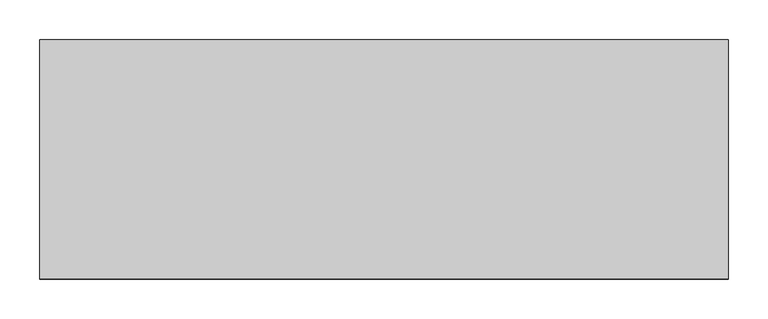
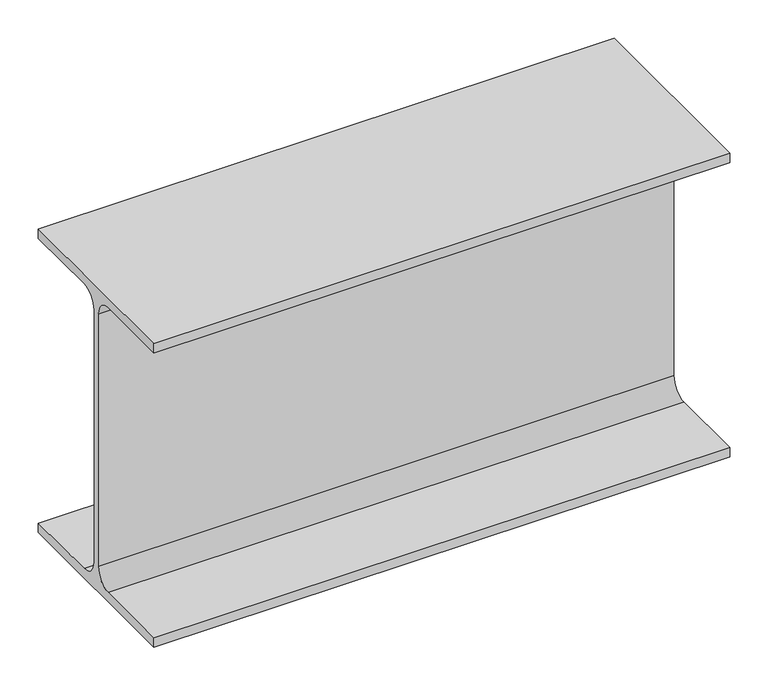
"""IFC4 building model written with IfcOpenShell, lengths in millimetres: beam geometry, 0912_Steel Framing_H-KSD3502 : H_SB_ASB_H-482x300x11x15."""

from ifc_helpers import new_model, si_unit, point, frame, frame_2d, origin, place, context, project, spatial, polyline, circle_curve, trimmed, segment, composite_curve, outline, extrude, source, transform, mapped, element, save


def beam_93cadcc3(model_context):
    return source(origin(), model_context, "Body", "SweptSolid", [
        extrude(outline(composite_curve([segment(polyline([(150.0, -226.0), (150.0, -241.0), (-150.0, -241.0), (-150.0, -226.0), (-31.5, -226.0)]), True, "CONTINUOUS"), segment(trimmed(circle_curve(frame_2d((-31.5, -200.0)), 26.0), [point((-31.5, -226.0))], [point((-5.5, -200.0))], True, "CARTESIAN"), True, "CONTINUOUS"), segment(polyline([(-5.5, -200.0), (-5.5, 200.0)]), True, "CONTINUOUS"), segment(trimmed(circle_curve(frame_2d((-31.5, 200.0)), 26.0), [point((-5.5, 200.0))], [point((-31.5, 226.0))], True, "CARTESIAN"), True, "CONTINUOUS"), segment(polyline([(-31.5, 226.0), (-150.0, 226.0), (-150.0, 241.0), (150.0, 241.0), (150.0, 226.0), (31.5, 226.0)]), True, "CONTINUOUS"), segment(trimmed(circle_curve(frame_2d((31.5, 200.0)), 26.0), [point((31.5, 226.0))], [point((5.5, 200.0))], True, "CARTESIAN"), True, "CONTINUOUS"), segment(polyline([(5.5, 200.0), (5.5, -200.0)]), True, "CONTINUOUS"), segment(trimmed(circle_curve(frame_2d((31.5, -200.0)), 26.0), [point((5.5, -200.0))], [point((31.5, -226.0))], True, "CARTESIAN"), True, "CONTINUOUS"), segment(polyline([(31.5, -226.0), (150.0, -226.0)]), True, "CONTINUOUS")], self_intersect=False)), frame((-431.8, 0.0, 0.0), z_axis=(1.0, 0.0, 0.0), x_axis=(0.0, 1.0, 0.0)), (0.0, 0.0, 1.0), 863.6),
    ])


if __name__ == "__main__":
    model = new_model("IFC4")
    model_context = context("Model", 3, world=origin())
    ifc_project = project(units=[si_unit("LENGTHUNIT", "METRE", prefix="MILLI")], contexts=[model_context])
    site = spatial("IfcSite", under=ifc_project)
    building = spatial("IfcBuilding", under=site)
    placement = place(None, origin())
    beam_shape = beam_93cadcc3(model_context)
    element("IfcBeam", 1, ObjectType="0912_Steel Framing_H-KSD3502 : H_SB_ASB_H-482x300x11x15", at=placement, inside=building, context=model_context, shape_type="MappedRepresentation", body=[
        mapped(beam_shape, transform((0.0, 0.0, 0.0), x_axis=(1.0, 0.0, 0.0), y_axis=(0.0, 1.0, 0.0), z_axis=(0.0, 0.0, 1.0))),
    ])
    save(model, "model.ifc")

# Revit data of these elements
# Type "0912_Steel Framing_H-KSD3502 : H_SB_ASB_H-482x300x11x15"
#   H_WM Code_1 = "S01AA001-00001 | Main Steel Structure Fabrication Work | Shelter/Building | Heavy Steel - Standard (Weight≥90KG/M) | Material: (   )"
#   H_WM Code_2 = "S03AA027-00001 | Main Steel Structure Erection Work | Shelter/Building | Heavy Steel (Weight≥90KG/M) | Material: (   )"
#   H_WM Code_3 = "S01AA010-00001 | Main Steel Structure Fabrication Work | Shelter/Building | Steel Painting/Coating | for Non-Fireproofed Steel Surface, Surface Preparation, Primer, Second & Final Coat | Material: (   )"
#   H_Q'ty Cal Type Tag = "SB-Q2"
#   Width = 30.0 cm
#   Web Thickness = 1.1 cm
#   Web Fillet = 2.6 cm
#   Warping Constant = 3680000.0 cm⁶
#   W = 0
#   Torsional Moment of Inertia = 88.2192 cm⁴
#   Section Area = 145.5 cm²
#   Plastic Modulus weak axis = 695.0 cm³
#   Plastic Modulus strong axis = 2790.0 cm³
#   Perimeter = 2.10 m²/m
#   Nominal Weight = 114.00 kgf/m
#   Moment of Inertia weak axis = 6760.00 cm⁴
#   Moment of Inertia strong axis = 60400.00 cm⁴
#   Height = 48.2 cm
#   Flange Thickness = 1.5 cm
#   Elastic Modulus weak axis = 451.0 cm³
#   Elastic Modulus strong axis = 2500.0 cm³
#   Centroid Vertical = 24.1 cm
#   Centroid Horizontal = 15.0 cm
#   Ix = 604000000
#   Length [instance default] = 1.5240 m
#   Zx = 2790000
#   b = 0.3000 m
#   h = 0.4820 m
#   r = 0.0260 m
#   s = 0.0110 m
#   t = 0.0150 m
#   A = 0.01455 m²
#   Structural Material [instance default] = Steel, 45-345
#   Assembly Code = ""
# Element 1 (IfcBeam, "0912_Steel Framing_H-KSD3502 : H_SB_ASB_H-482x300x11x15")
#   Structural Material = none
# Materials
#   "Steel, 45-345": class "Metal", colour RGB 189 187 185, transparency 0, Description = "Steel 345 MPa", Cost = 0
